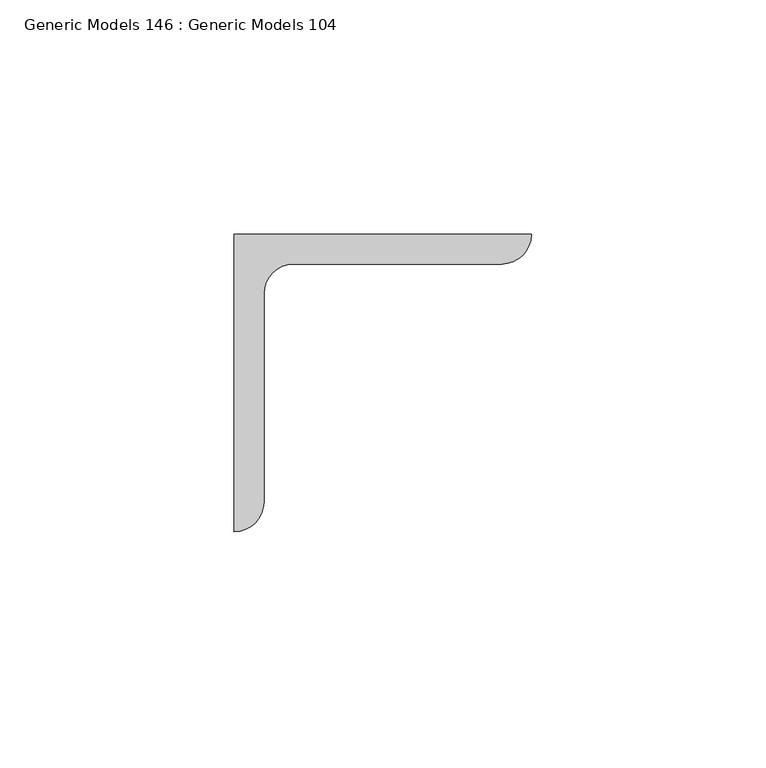
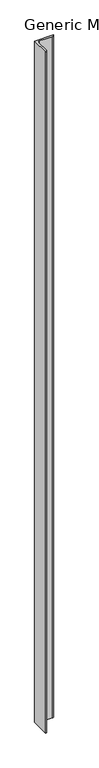
"""IFC4 building model written with IfcOpenShell, lengths in millimetres: proxy geometry, Generic Models 146 : Generic Models 104."""

from ifc_helpers import new_model, si_unit, point, frame, frame_2d, origin, place, context, project, spatial, polyline, circle_curve, trimmed, segment, composite_curve, outline, extrude, source, transform, mapped, element, save


def generic_models_146_generic_models_104_6500cd60(model_context):
    return source(origin(), model_context, "Body", "SweptSolid", [
        extrude(outline(composite_curve([segment(polyline([(35362.35773, 41071.1196612), (35425.85773, 41071.1196612)]), True, "CONTINUOUS"), segment(trimmed(circle_curve(frame_2d((35419.50773, 41071.1196612)), 6.35), [point((35425.85773, 41071.1196612))], [point((35419.50773, 41064.7696612))], False, "CARTESIAN"), True, "CONTINUOUS"), segment(polyline([(35419.50773, 41064.7696612), (35375.05773, 41064.7696612)]), True, "CONTINUOUS"), segment(trimmed(circle_curve(frame_2d((35375.05773, 41058.4196612)), 6.35), [point((35375.05773, 41064.7696612))], [point((35368.70773, 41058.4196612))], True, "CARTESIAN"), True, "CONTINUOUS"), segment(polyline([(35368.70773, 41058.4196612), (35368.70773, 41013.9696612)]), True, "CONTINUOUS"), segment(trimmed(circle_curve(frame_2d((35362.35773, 41013.9696612)), 6.35), [point((35368.70773, 41013.9696612))], [point((35362.35773, 41007.6196612))], False, "CARTESIAN"), True, "CONTINUOUS"), segment(polyline([(35362.35773, 41007.6196612), (35362.35773, 41071.1196612)]), True, "CONTINUOUS")], self_intersect=False)), frame((0.0, 0.0, 266407.9), z_axis=(0.0, 0.0, 1.0), x_axis=(1.0, 0.0, 0.0)), (0.0, 0.0, 1.0), 2432.1044757),
    ])


if __name__ == "__main__":
    model = new_model("IFC4")
    model_context = context("Model", 3, world=origin())
    ifc_project = project(units=[si_unit("LENGTHUNIT", "METRE", prefix="MILLI")], contexts=[model_context])
    site = spatial("IfcSite", under=ifc_project)
    building = spatial("IfcBuilding", under=site)
    placement = place(None, origin())
    generic_models_146_generic_models_104_shape = generic_models_146_generic_models_104_6500cd60(model_context)
    element("IfcBuildingElementProxy", 1, Name="Generic Models 146 : Generic Models 104", ObjectType="Generic Models 146 : Generic Models 104", at=placement, inside=building, context=model_context, shape_type="MappedRepresentation", body=[
        mapped(generic_models_146_generic_models_104_shape, transform((0.0, 0.0, 0.0), x_axis=(1.0, 0.0, 0.0), y_axis=(0.0, 1.0, 0.0), z_axis=(0.0, 0.0, 1.0))),
    ])
    save(model, "model.ifc")

# Revit data of these elements
# Element 1 (IfcBuildingElementProxy, "Generic Models 146 : Generic Models 104")
#   Materials on its faces: "(2) BACK/BACK GALVANIZED ANGLES (2) L2 1/2 X 2 1/2 X 1/4\")"
# Materials
#   "(2) BACK/BACK GALVANIZED ANGLES (2) L2 1/2 X 2 1/2 X 1/4\")": class "Unassigned", colour RGB 211 211 211, transparency 0, Cost = 0
